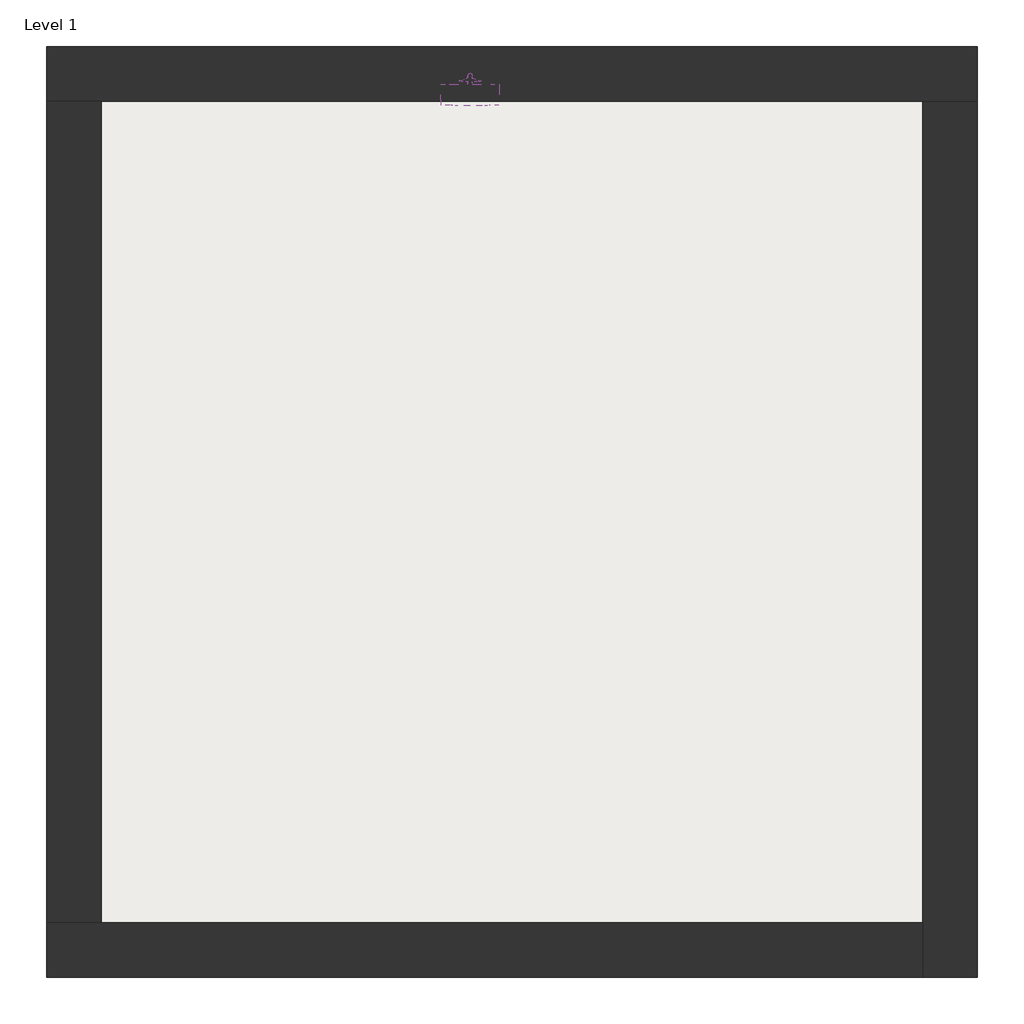
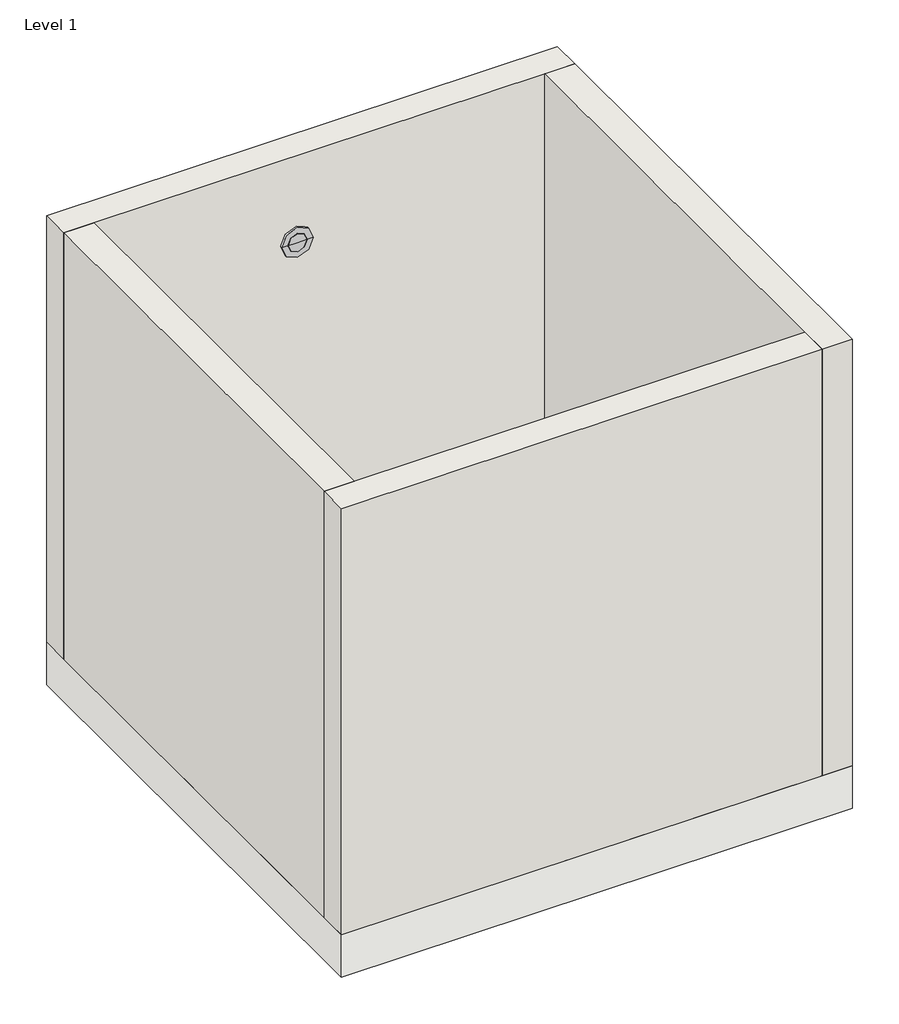
# One storey: 4 walls, 1 proxy, 1 slab.
"""IFC4 building model written with IfcOpenShell, lengths in millimetres."""

import ifcopenshell
import ifcopenshell.guid

model = None  # the IFC model being written
_history = None  # IfcOwnerHistory: only IFC2X3 demands one
_inside = {}  # id of a spatial element -> (the spatial element, [elements in it])
_under = {}  # id of a project, library or spatial element -> (it, [spatial elements below it])
_declared = {}  # id of a project -> (the project, [libraries it declares])
_typed = {}  # id of a type object -> (the type object, [elements of that type])
_made_of = {}  # id of a material, layer set ... -> (it, [elements and type objects made of it])


def new_model(schema):
    """Start an empty IFC model of exactly this schema.

    Asked for "IFC4X3", IfcOpenShell would pick the latest addendum, in which some entities
    have other attributes; the version numbers below select the first issue.
    IFC2X3 requires an IfcOwnerHistory on every rooted entity: one is made here for all.
    """
    global model, _history
    if schema == "IFC4X3":
        model = ifcopenshell.file(schema_version=(4, 3, 0, 0))
    else:
        model = ifcopenshell.file(schema=schema)
    _inside.clear()
    _under.clear()
    _declared.clear()
    _typed.clear()
    _made_of.clear()
    _history = None
    if model.schema == "IFC2X3":
        org = make("IfcOrganization", Name="unknown")
        user = make(
            "IfcPersonAndOrganization",
            ThePerson=make("IfcPerson", FamilyName="unknown"),
            TheOrganization=org,
        )
        app = make(
            "IfcApplication",
            ApplicationDeveloper=org,
            Version="unknown",
            ApplicationFullName="unknown",
            ApplicationIdentifier="unknown",
        )
        _history = make(
            "IfcOwnerHistory",
            OwningUser=user,
            OwningApplication=app,
            ChangeAction="ADDED",
            CreationDate=0,
        )
    return model


def make(cls, **values):
    """One entity of the class cls with the attributes given. An attribute that is None is left unset."""
    return model.create_entity(
        cls, **{name: value for name, value in values.items() if value is not None}
    )


def rooted(cls, **values):
    """An entity with a GlobalId (a new one), such as an element, a storey or a relation."""
    return make(cls, GlobalId=ifcopenshell.guid.new(), OwnerHistory=_history, **values)


def si_unit(unit_type, name, prefix=None):
    """IfcSIUnit, for example si_unit("LENGTHUNIT", "METRE", prefix="MILLI")."""
    return make("IfcSIUnit", UnitType=unit_type, Prefix=prefix, Name=name)


def assignment(units):
    """IfcUnitAssignment: the units of a project."""
    return None if units is None else make("IfcUnitAssignment", Units=units)


def point(xyz):
    """IfcCartesianPoint."""
    return None if xyz is None else make("IfcCartesianPoint", Coordinates=xyz)


def direction(xyz):
    """IfcDirection."""
    return None if xyz is None else make("IfcDirection", DirectionRatios=xyz)


def frame(location, z_axis=None, x_axis=None):
    """IfcAxis2Placement3D, a coordinate frame: its origin and axes. An axis left out is left unset."""
    return make(
        "IfcAxis2Placement3D",
        Location=point(location),
        Axis=direction(z_axis),
        RefDirection=direction(x_axis),
    )


def origin():
    """The frame at (0, 0, 0) with its axes left unset."""
    return frame((0.0, 0.0, 0.0))


def origin_with_axes():
    """The frame at (0, 0, 0) with the z axis (0, 0, 1) and the x axis (1, 0, 0) written out."""
    return frame((0.0, 0.0, 0.0), z_axis=(0.0, 0.0, 1.0), x_axis=(1.0, 0.0, 0.0))


def place(relative_to, where):
    """IfcLocalPlacement: puts the frame where relative to a parent placement (None: the world)."""
    return make(
        "IfcLocalPlacement", PlacementRelTo=relative_to, RelativePlacement=where
    )


def context(
    kind, dimensions, precision=None, world=None, true_north=None, identifier=None
):
    """IfcGeometricRepresentationContext, for example the 3D "Model" context."""
    return make(
        "IfcGeometricRepresentationContext",
        ContextIdentifier=identifier,
        ContextType=kind,
        CoordinateSpaceDimension=dimensions,
        Precision=precision,
        WorldCoordinateSystem=world,
        TrueNorth=true_north,
    )


def project(units=None, contexts=None):
    """IfcProject with its units and contexts."""
    return rooted(
        "IfcProject",
        Name="project",
        RepresentationContexts=contexts,
        UnitsInContext=assignment(units),
    )


def spatial(cls, under=None, at=None, **own):
    """A site, building, storey or space (cls), placed at a placement, below another one or the project."""
    s = rooted(cls, ObjectPlacement=at, **own)
    if under is not None:
        _under.setdefault(under.id(), (under, []))[1].append(s)
    return s


def polyline(points):
    """IfcPolyline through the points."""
    return make("IfcPolyline", Points=[point(p) for p in points])


def circle_curve(where, radius):
    """IfcCircle in the frame where."""
    return make("IfcCircle", Position=where, Radius=radius)


def ellipse_curve(where, semi_axis1, semi_axis2):
    """IfcEllipse in the frame where."""
    return make(
        "IfcEllipse", Position=where, SemiAxis1=semi_axis1, SemiAxis2=semi_axis2
    )


def trimmed(basis, trim1, trim2, sense, master):
    """IfcTrimmedCurve: the piece of a basis curve between two trims."""
    return make(
        "IfcTrimmedCurve",
        BasisCurve=basis,
        Trim1=trim1,
        Trim2=trim2,
        SenseAgreement=sense,
        MasterRepresentation=master,
    )


def outline(outer, holes=None, kind="AREA"):
    """IfcArbitraryClosedProfileDef: a profile drawn as a closed curve; with holes, ...WithVoids."""
    if holes is None:
        return make("IfcArbitraryClosedProfileDef", ProfileType=kind, OuterCurve=outer)
    return make(
        "IfcArbitraryProfileDefWithVoids",
        ProfileType=kind,
        OuterCurve=outer,
        InnerCurves=holes,
    )


def extrude(swept, where, along, depth):
    """IfcExtrudedAreaSolid: the profile swept, set in the frame where, extruded along a direction by depth."""
    return make(
        "IfcExtrudedAreaSolid",
        SweptArea=swept,
        Position=where,
        ExtrudedDirection=direction(along),
        Depth=depth,
    )


def faces_of(points, faces, orient=None, outer=None):
    """IfcFace entities. A face is a list of loops; a loop is a list of indices into points, from 0.

    orient and outer hold one flag for each loop. By default every Orientation is true, the
    first loop of a face is its IfcFaceOuterBound and the others are IfcFaceBound.
    """
    made = []
    for i, loops in enumerate(faces):
        bounds = []
        for j, loop in enumerate(loops):
            is_outer = j == 0 if outer is None else outer[i][j]
            bounds.append(
                make(
                    "IfcFaceOuterBound" if is_outer else "IfcFaceBound",
                    Bound=make("IfcPolyLoop", Polygon=[points[k] for k in loop]),
                    Orientation=True if orient is None else orient[i][j],
                )
            )
        made.append(make("IfcFace", Bounds=bounds))
    return made


def faceted_brep(points, faces, orient=None, outer=None, voids=None):
    """IfcFacetedBrep: a solid bounded by flat faces; with voids (closed shells), ...WithVoids."""
    shared = [point(p) for p in points]
    hull = make("IfcClosedShell", CfsFaces=faces_of(shared, faces, orient, outer))
    if voids is None:
        return make("IfcFacetedBrep", Outer=hull)
    return make(
        "IfcFacetedBrepWithVoids",
        Outer=hull,
        Voids=[
            make(cls, CfsFaces=faces_of(shared, fs, o, b)) for cls, fs, o, b in voids
        ],
    )


def shape(context_of_items, identifier, shape_type, items):
    """IfcShapeRepresentation: the items that make up one representation, for example the "Body"."""
    return make(
        "IfcShapeRepresentation",
        ContextOfItems=context_of_items,
        RepresentationIdentifier=identifier,
        RepresentationType=shape_type,
        Items=items,
    )


def source(mapping_origin, context_of_items, identifier, shape_type, items):
    """IfcRepresentationMap: a shape defined once, which mapped items show again and again."""
    return make(
        "IfcRepresentationMap",
        MappingOrigin=mapping_origin,
        MappedRepresentation=shape(context_of_items, identifier, shape_type, items),
    )


def transform(
    local_origin,
    x_axis=None,
    y_axis=None,
    z_axis=None,
    scale=None,
    scale2=None,
    scale3=None,
    uniform=True,
):
    """IfcCartesianTransformationOperator3D, or its non-uniform kind. x_axis, y_axis, z_axis: its Axis1, 2, 3."""
    if uniform:
        return make(
            "IfcCartesianTransformationOperator3D",
            Axis1=direction(x_axis),
            Axis2=direction(y_axis),
            LocalOrigin=point(local_origin),
            Scale=scale,
            Axis3=direction(z_axis),
        )
    return make(
        "IfcCartesianTransformationOperator3DnonUniform",
        Axis1=direction(x_axis),
        Axis2=direction(y_axis),
        LocalOrigin=point(local_origin),
        Scale=scale,
        Axis3=direction(z_axis),
        Scale2=scale2,
        Scale3=scale3,
    )


def mapped(mapping_source, mapping_target):
    """IfcMappedItem: shows the shape of a source again, moved by a transform."""
    return make(
        "IfcMappedItem", MappingSource=mapping_source, MappingTarget=mapping_target
    )


def made_of(thing, what):
    """Note that an element or type object is made of a material, layer set ...; save() writes the relation."""
    if what is not None:
        _made_of.setdefault(what.id(), (what, []))[1].append(thing)
    return thing


def element(
    cls,
    number,
    at=None,
    inside=None,
    cuts=None,
    type_object=None,
    material=None,
    context=None,
    identifier="Body",
    shape_type=None,
    held_by="IfcProductDefinitionShape",
    body=None,
    shapes=None,
    **own,
):
    """One element of the class cls, such as IfcWall. Its Tag is "e" and its number.

    at: its placement. inside: the storey or other place that contains it. cuts: it is an
    opening in that element (IfcRelVoidsElement). A single representation is given by context,
    identifier, shape_type and body (its items); several are given by shapes. held_by: the class
    of the entity that holds the representations. save() writes the other relations.
    """
    e = rooted(cls, Tag="e%d" % number, ObjectPlacement=at, **own)
    if body is not None:
        shapes = [shape(context, identifier, shape_type, body)]
    if shapes is not None:
        e.Representation = make(held_by, Representations=shapes)
    if inside is not None:
        _inside.setdefault(inside.id(), (inside, []))[1].append(e)
    if cuts is not None:
        rooted(
            "IfcRelVoidsElement", RelatingBuildingElement=cuts, RelatedOpeningElement=e
        )
    if type_object is not None:
        _typed.setdefault(type_object.id(), (type_object, []))[1].append(e)
    return made_of(e, material)


def aggregate(whole, parts):
    """IfcRelAggregates: a whole, such as a stair, and the parts it consists of."""
    return rooted("IfcRelAggregates", RelatingObject=whole, RelatedObjects=parts)


def save(model, path):
    """Write the relations noted so far, then the file.

    IfcRelAggregates (storeys below a building ...), IfcRelContainedInSpatialStructure (elements
    in a storey), IfcRelDefinesByType, IfcRelAssociatesMaterial and IfcRelDeclares: one each for
    every whole, place, type object, material and project.
    """
    for whole, parts in _under.values():
        aggregate(whole, parts)
    for where, things in _inside.values():
        rooted(
            "IfcRelContainedInSpatialStructure",
            RelatedElements=things,
            RelatingStructure=where,
        )
    for kind, things in _typed.values():
        rooted("IfcRelDefinesByType", RelatedObjects=things, RelatingType=kind)
    for what, things in _made_of.values():
        rooted("IfcRelAssociatesMaterial", RelatedObjects=things, RelatingMaterial=what)
    for by, libraries in _declared.values():
        rooted("IfcRelDeclares", RelatingContext=by, RelatedDefinitions=libraries)
    model.write(path)


def plane_surface(at):
    """IfcPlane: the flat surface through the origin of the frame at, square to its z axis."""
    return make("IfcPlane", Position=at)


def cylinder_surface(at, radius):
    """IfcCylindricalSurface: all points at the distance radius from the z axis of the frame at."""
    return make("IfcCylindricalSurface", Position=at, Radius=radius)


def revolved_surface(curve, axis_point, axis_direction):
    """IfcSurfaceOfRevolution: the curve turned about the line through axis_point along axis_direction."""
    return make(
        "IfcSurfaceOfRevolution",
        SweptCurve=make("IfcArbitraryOpenProfileDef", ProfileType="CURVE", Curve=curve),
        AxisPosition=make("IfcAxis1Placement", Location=point(axis_point), Axis=direction(axis_direction)),
    )


def spline_curve(degree, points, multiplicities, knots, weights=None):
    """IfcBSplineCurveWithKnots; with weights, IfcRationalBSplineCurveWithKnots."""
    own = dict(
        Degree=degree,
        ControlPointsList=[point(p) for p in points],
        CurveForm="UNSPECIFIED",
        ClosedCurve=False,
        SelfIntersect=False,
        KnotMultiplicities=multiplicities,
        Knots=knots,
        KnotSpec="UNSPECIFIED",
    )
    if weights is None:
        return make("IfcBSplineCurveWithKnots", **own)
    return make("IfcRationalBSplineCurveWithKnots", WeightsData=weights, **own)


def advanced_brep(points, edges, surfaces, faces):
    """IfcAdvancedBrep: a solid bounded by faces that lie on surfaces and meet in shared edges.

    An edge is (start, end): straight between two places in points (the first is 0);
    or (start, end, curve); or (start, end, curve, False) where it runs against its curve.
    A face is (place in surfaces, loops), or (place, loops, False) where it looks against
    its surface's normal. A loop lists edges by number (the first is 1), with a minus sign
    where the edge is run from its end to its start. The first loop is the outer one.
    """
    corners = [point(p) for p in points]
    vertices = [make("IfcVertexPoint", VertexGeometry=c) for c in corners]
    made = []
    for start, end, *more in edges:
        made.append(
            make(
                "IfcEdgeCurve",
                EdgeStart=vertices[start],
                EdgeEnd=vertices[end],
                EdgeGeometry=more[0] if more else make("IfcPolyline", Points=[corners[start], corners[end]]),
                SameSense=more[1] if len(more) > 1 else True,
            )
        )
    hull = []
    for where, loops, *sense in faces:
        bounds = []
        for j, loop in enumerate(loops):
            ring = [make("IfcOrientedEdge", EdgeElement=made[abs(k) - 1], Orientation=k > 0) for k in loop]
            bounds.append(
                make(
                    "IfcFaceOuterBound" if j == 0 else "IfcFaceBound",
                    Bound=make("IfcEdgeLoop", EdgeList=ring),
                    Orientation=True,
                )
            )
        hull.append(make("IfcAdvancedFace", Bounds=bounds, FaceSurface=surfaces[where], SameSense=sense[0] if sense else True))
    return make("IfcAdvancedBrep", Outer=make("IfcClosedShell", CfsFaces=hull))


def mechanical_equipment_c477e944(model_context):
    return source(origin(), model_context, "Body", "AdvancedBrep", [
        advanced_brep(
        [(121.9974459, -0.199999, 2400.0), (128.0025541, -0.199999, 2400.0), (128.0025541, -2.4999994, 2400.0), (121.9974459, -2.4999994, 2400.0), (119.1058972, -0.199999, 2400.0), (130.8941028, -0.199999, 2400.0), (119.1058972, 4.9999993, 2400.0), (130.8941028, 4.9999993, 2400.0), (116.7764643, 4.9999993, 2400.0), (133.2235357, 4.9999993, 2400.0), (116.7764643, 10.0000007, 2400.0), (133.2235357, 10.0000007, 2400.0), (117.7564219, 10.0000007, 2400.0), (132.2435781, 10.0000007, 2400.0), (117.7564219, 13.8000004, 2400.0), (132.2435781, 13.8000004, 2400.0), (116.0662237, 13.8000004, 2400.0), (133.9337763, 13.8000004, 2400.0), (114.7691944, 15.1302816, 2400.0), (135.2308056, 15.1302816, 2400.0), (114.7691944, 15.9854344, 2400.0), (135.2308056, 15.9854344, 2400.0), (111.2784266, 15.9854344, 2400.0), (138.7215734, 15.9854344, 2400.0), (90.472179, 26.7999995, 2400.0), (159.527821, 26.7999995, 2400.0), (87.519154, 26.7999995, 2400.0), (162.480846, 26.7999995, 2400.0), (86.2128962, 25.9940284, 2400.0), (163.7871038, 25.9940284, 2400.0), (86.2128962, 24.0999996, 2400.0), (163.7871038, 24.0999996, 2400.0), (85.0392013, 24.0999996, 2400.0), (164.9607987, 24.0999996, 2400.0), (85.0392013, 25.9940284, 2400.0), (164.9607987, 25.9940284, 2400.0), (87.0451729, 28.0, 2400.0), (162.9548271, 28.0, 2400.0), (119.1058972, 28.0, 2400.0), (130.8941028, 28.0, 2400.0), (119.1058972, 32.5000002, 2400.0), (130.8941028, 32.5000002, 2400.0), (116.7764643, 32.5000002, 2400.0), (133.2235357, 32.5000002, 2400.0), (116.7764643, 37.4999999, 2400.0), (133.2235357, 37.4999999, 2400.0), (18.250711, 37.4999999, 2400.0), (231.749289, 37.4999999, 2400.0), (19.5859291, 113.9945916, 2400.0), (230.4140709, 113.9945916, 2400.0), (59.5859291, 113.9945916, 2400.0), (190.4140709, 113.9945916, 2400.0), (61.724849, 116.1335115, 2400.0), (188.275151, 116.1335115, 2400.0), (125.0, 116.1335115, 2400.0), (125.0, -2.4999994, 2400.0)],
        [
            (0, 1, circle_curve(frame((125.0, -0.199999, 2400.0), z_axis=(0.0, -1.0, 0.0), x_axis=(1.0, 0.0, 0.0)), 3.0025541)),
            (1, 2),
            (2, 3, circle_curve(frame((125.0, -2.4999994, 2400.0), z_axis=(0.0, 1.0, 0.0), x_axis=(1.0, 0.0, 0.0)), 3.0025541)),
            (3, 0),
            (1, 0, circle_curve(frame((125.0, -0.199999, 2400.0), z_axis=(0.0, -1.0, 0.0), x_axis=(1.0, 0.0, 0.0)), 3.0025541)),
            (3, 2, circle_curve(frame((125.0, -2.4999994, 2400.0), z_axis=(0.0, 1.0, 0.0), x_axis=(1.0, 0.0, 0.0)), 3.0025541)),
            (4, 5, circle_curve(frame((125.0, -0.199999, 2400.0), z_axis=(0.0, -1.0, 0.0), x_axis=(1.0, 0.0, 0.0)), 5.8941028)),
            (5, 1),
            (0, 4),
            (5, 4, circle_curve(frame((125.0, -0.199999, 2400.0), z_axis=(0.0, -1.0, 0.0), x_axis=(1.0, 0.0, 0.0)), 5.8941028)),
            (6, 7, circle_curve(frame((125.0, 4.9999993, 2400.0), z_axis=(0.0, -1.0, 0.0), x_axis=(1.0, 0.0, 0.0)), 5.8941028)),
            (7, 5),
            (4, 6),
            (7, 6, circle_curve(frame((125.0, 4.9999993, 2400.0), z_axis=(0.0, -1.0, 0.0), x_axis=(1.0, 0.0, 0.0)), 5.8941028)),
            (8, 9, circle_curve(frame((125.0, 4.9999993, 2400.0), z_axis=(0.0, -1.0, 0.0), x_axis=(1.0, 0.0, 0.0)), 8.2235357)),
            (9, 7),
            (6, 8),
            (9, 8, circle_curve(frame((125.0, 4.9999993, 2400.0), z_axis=(0.0, -1.0, 0.0), x_axis=(1.0, 0.0, 0.0)), 8.2235357)),
            (10, 11, circle_curve(frame((125.0, 10.0000007, 2400.0), z_axis=(0.0, -1.0, 0.0), x_axis=(1.0, 0.0, 0.0)), 8.2235357)),
            (11, 9),
            (8, 10),
            (11, 10, circle_curve(frame((125.0, 10.0000007, 2400.0), z_axis=(0.0, -1.0, 0.0), x_axis=(1.0, 0.0, 0.0)), 8.2235357)),
            (12, 13, circle_curve(frame((125.0, 10.0000007, 2400.0), z_axis=(0.0, -1.0, 0.0), x_axis=(1.0, 0.0, 0.0)), 7.2435781)),
            (13, 11),
            (10, 12),
            (13, 12, circle_curve(frame((125.0, 10.0000007, 2400.0), z_axis=(0.0, -1.0, 0.0), x_axis=(1.0, 0.0, 0.0)), 7.2435781)),
            (14, 15, circle_curve(frame((125.0, 13.8000004, 2400.0), z_axis=(0.0, -1.0, 0.0), x_axis=(1.0, 0.0, 0.0)), 7.2435781)),
            (15, 13),
            (12, 14),
            (15, 14, circle_curve(frame((125.0, 13.8000004, 2400.0), z_axis=(0.0, -1.0, 0.0), x_axis=(1.0, 0.0, 0.0)), 7.2435781)),
            (16, 17, circle_curve(frame((125.0, 13.8000004, 2400.0), z_axis=(0.0, -1.0, 0.0), x_axis=(1.0, 0.0, 0.0)), 8.9337763)),
            (17, 15),
            (14, 16),
            (17, 16, circle_curve(frame((125.0, 13.8000004, 2400.0), z_axis=(0.0, -1.0, 0.0), x_axis=(1.0, 0.0, 0.0)), 8.9337763)),
            (18, 19, circle_curve(frame((125.0, 15.1302816, 2400.0), z_axis=(0.0, -1.0, 0.0), x_axis=(1.0, 0.0, 0.0)), 10.2308056)),
            (19, 17, spline_curve(3, [(135.2308056, 15.1302816, 2400.0), (135.18031757, 14.408269131, 2400.0), (134.747974442, 13.964842091, 2400.0), (133.9337763, 13.8000004, 2400.0)], [4, 4], [0.0, 0.003825031864308585])),
            (16, 18, spline_curve(3, [(116.0662237, 13.8000004, 2400.0), (115.252025558, 13.964842091, 2400.0), (114.81968243, 14.408269131, 2400.0), (114.7691944, 15.1302816, 2400.0)], [4, 4], [0.0, 0.003825031864308585])),
            (19, 18, circle_curve(frame((125.0, 15.1302816, 2400.0), z_axis=(0.0, -1.0, 0.0), x_axis=(1.0, 0.0, 0.0)), 10.2308056)),
            (20, 21, circle_curve(frame((125.0, 15.9854344, 2400.0), z_axis=(0.0, -1.0, 0.0), x_axis=(1.0, 0.0, 0.0)), 10.2308056)),
            (21, 19),
            (18, 20),
            (21, 20, circle_curve(frame((125.0, 15.9854344, 2400.0), z_axis=(0.0, -1.0, 0.0), x_axis=(1.0, 0.0, 0.0)), 10.2308056)),
            (22, 23, circle_curve(frame((125.0, 15.9854344, 2400.0), z_axis=(0.0, -1.0, 0.0), x_axis=(1.0, 0.0, 0.0)), 13.7215734)),
            (23, 21),
            (20, 22),
            (23, 22, circle_curve(frame((125.0, 15.9854344, 2400.0), z_axis=(0.0, -1.0, 0.0), x_axis=(1.0, 0.0, 0.0)), 13.7215734)),
            (24, 25, circle_curve(frame((125.0, 26.7999995, 2400.0), z_axis=(0.0, -1.0, 0.0), x_axis=(1.0, 0.0, 0.0)), 34.527821)),
            (25, 23, spline_curve(3, [(159.527821, 26.7999995, 2400.0), (152.920328589, 20.192507089, 2400.0), (145.984912731, 16.587652064, 2400.0), (138.7215734, 15.9854344, 2400.0)], [4, 4], [0.0, 0.04037262450680565])),
            (22, 24, spline_curve(3, [(111.2784266, 15.9854344, 2400.0), (104.015087269, 16.587652064, 2400.0), (97.079671411, 20.192507089, 2400.0), (90.472179, 26.7999995, 2400.0)], [4, 4], [0.0, 0.04037262450680565])),
            (25, 24, circle_curve(frame((125.0, 26.7999995, 2400.0), z_axis=(0.0, -1.0, 0.0), x_axis=(1.0, 0.0, 0.0)), 34.527821)),
            (26, 27, circle_curve(frame((125.0, 26.7999995, 2400.0), z_axis=(0.0, -1.0, 0.0), x_axis=(1.0, 0.0, 0.0)), 37.480846)),
            (27, 25),
            (24, 26),
            (27, 26, circle_curve(frame((125.0, 26.7999995, 2400.0), z_axis=(0.0, -1.0, 0.0), x_axis=(1.0, 0.0, 0.0)), 37.480846)),
            (28, 29, circle_curve(frame((125.0, 25.9940284, 2400.0), z_axis=(0.0, -1.0, 0.0), x_axis=(1.0, 0.0, 0.0)), 38.7871038)),
            (29, 27, circle_curve(frame((162.7127782, 25.7143697, 2400.0), z_axis=(0.0, 0.0, 1.0), x_axis=(-1.0, 0.0, 0.0)), 1.1101281)),
            (26, 28, circle_curve(frame((87.2872218, 25.7143697, 2400.0), z_axis=(0.0, 0.0, 1.0), x_axis=(1.0, 0.0, 0.0)), 1.1101281)),
            (29, 28, circle_curve(frame((125.0, 25.9940284, 2400.0), z_axis=(0.0, -1.0, 0.0), x_axis=(1.0, 0.0, 0.0)), 38.7871038)),
            (30, 31, circle_curve(frame((125.0, 24.0999996, 2400.0), z_axis=(0.0, -1.0, 0.0), x_axis=(1.0, 0.0, 0.0)), 38.7871038)),
            (31, 29),
            (28, 30),
            (31, 30, circle_curve(frame((125.0, 24.0999996, 2400.0), z_axis=(0.0, -1.0, 0.0), x_axis=(1.0, 0.0, 0.0)), 38.7871038)),
            (32, 33, circle_curve(frame((125.0, 24.0999996, 2400.0), z_axis=(0.0, -1.0, 0.0), x_axis=(1.0, 0.0, 0.0)), 39.9607987)),
            (33, 31),
            (30, 32),
            (33, 32, circle_curve(frame((125.0, 24.0999996, 2400.0), z_axis=(0.0, -1.0, 0.0), x_axis=(1.0, 0.0, 0.0)), 39.9607987)),
            (34, 35, circle_curve(frame((125.0, 25.9940284, 2400.0), z_axis=(0.0, -1.0, 0.0), x_axis=(1.0, 0.0, 0.0)), 39.9607987)),
            (35, 33),
            (32, 34),
            (35, 34, circle_curve(frame((125.0, 25.9940284, 2400.0), z_axis=(0.0, -1.0, 0.0), x_axis=(1.0, 0.0, 0.0)), 39.9607987)),
            (36, 37, circle_curve(frame((125.0, 28.0, 2400.0), z_axis=(0.0, -1.0, 0.0), x_axis=(1.0, 0.0, 0.0)), 37.9548271)),
            (37, 35, circle_curve(frame((162.9548271, 25.9940284, 2400.0), z_axis=(0.0, 0.0, -1.0), x_axis=(-1.0, 0.0, 0.0)), 2.0059716)),
            (34, 36, circle_curve(frame((87.0451729, 25.9940284, 2400.0), z_axis=(0.0, 0.0, -1.0), x_axis=(1.0, 0.0, 0.0)), 2.0059716)),
            (37, 36, circle_curve(frame((125.0, 28.0, 2400.0), z_axis=(0.0, -1.0, 0.0), x_axis=(1.0, 0.0, 0.0)), 37.9548271)),
            (38, 39, circle_curve(frame((125.0, 28.0, 2400.0), z_axis=(0.0, -1.0, 0.0), x_axis=(1.0, 0.0, 0.0)), 5.8941028)),
            (39, 37),
            (36, 38),
            (39, 38, circle_curve(frame((125.0, 28.0, 2400.0), z_axis=(0.0, -1.0, 0.0), x_axis=(1.0, 0.0, 0.0)), 5.8941028)),
            (40, 41, circle_curve(frame((125.0, 32.5000002, 2400.0), z_axis=(0.0, -1.0, 0.0), x_axis=(1.0, 0.0, 0.0)), 5.8941028)),
            (41, 39),
            (38, 40),
            (41, 40, circle_curve(frame((125.0, 32.5000002, 2400.0), z_axis=(0.0, -1.0, 0.0), x_axis=(1.0, 0.0, 0.0)), 5.8941028)),
            (42, 43, circle_curve(frame((125.0, 32.5000002, 2400.0), z_axis=(0.0, -1.0, 0.0), x_axis=(1.0, 0.0, 0.0)), 8.2235357)),
            (43, 41),
            (40, 42),
            (43, 42, circle_curve(frame((125.0, 32.5000002, 2400.0), z_axis=(0.0, -1.0, 0.0), x_axis=(1.0, 0.0, 0.0)), 8.2235357)),
            (44, 45, circle_curve(frame((125.0, 37.4999999, 2400.0), z_axis=(0.0, -1.0, 0.0), x_axis=(1.0, 0.0, 0.0)), 8.2235357)),
            (45, 43),
            (42, 44),
            (45, 44, circle_curve(frame((125.0, 37.4999999, 2400.0), z_axis=(0.0, -1.0, 0.0), x_axis=(1.0, 0.0, 0.0)), 8.2235357)),
            (46, 47, circle_curve(frame((125.0, 37.4999999, 2400.0), z_axis=(0.0, -1.0, 0.0), x_axis=(1.0, 0.0, 0.0)), 106.749289)),
            (47, 45),
            (44, 46),
            (47, 46, circle_curve(frame((125.0, 37.4999999, 2400.0), z_axis=(0.0, -1.0, 0.0), x_axis=(1.0, 0.0, 0.0)), 106.749289)),
            (48, 49, circle_curve(frame((125.0, 113.9945916, 2400.0), z_axis=(0.0, -1.0, 0.0), x_axis=(1.0, 0.0, 0.0)), 105.4140709)),
            (49, 47),
            (46, 48),
            (49, 48, circle_curve(frame((125.0, 113.9945916, 2400.0), z_axis=(0.0, -1.0, 0.0), x_axis=(1.0, 0.0, 0.0)), 105.4140709)),
            (50, 51, circle_curve(frame((125.0, 113.9945916, 2400.0), z_axis=(0.0, -1.0, 0.0), x_axis=(1.0, 0.0, 0.0)), 65.4140709)),
            (51, 49),
            (48, 50),
            (51, 50, circle_curve(frame((125.0, 113.9945916, 2400.0), z_axis=(0.0, -1.0, 0.0), x_axis=(1.0, 0.0, 0.0)), 65.4140709)),
            (52, 53, circle_curve(frame((125.0, 116.1335115, 2400.0), z_axis=(0.0, -1.0, 0.0), x_axis=(1.0, 0.0, 0.0)), 63.275151)),
            (53, 51),
            (50, 52),
            (53, 52, circle_curve(frame((125.0, 116.1335115, 2400.0), z_axis=(0.0, -1.0, 0.0), x_axis=(1.0, 0.0, 0.0)), 63.275151)),
            (54, 53),
            (52, 54),
            (2, 55),
            (55, 3),
        ],
        [
            cylinder_surface(frame((125.0, -65.0, 2400.0), z_axis=(0.0, 1.0, 0.0), x_axis=(1.0, 0.0, 0.0)), 3.0025541),
            plane_surface(frame((125.0, -0.199999, 2400.0), z_axis=(0.0, -1.0, 0.0), x_axis=(1.0, 0.0, 0.0))),
            cylinder_surface(frame((125.0, -65.0, 2400.0), z_axis=(0.0, 1.0, 0.0), x_axis=(1.0, 0.0, 0.0)), 5.8941028),
            plane_surface(frame((125.0, 4.9999993, 2400.0), z_axis=(0.0, -1.0, 0.0), x_axis=(1.0, 0.0, 0.0))),
            cylinder_surface(frame((125.0, -65.0, 2400.0), z_axis=(0.0, 1.0, 0.0), x_axis=(1.0, 0.0, 0.0)), 8.2235357),
            plane_surface(frame((125.0, 10.0000007, 2400.0), z_axis=(0.0, 1.0, 0.0), x_axis=(1.0, 0.0, 0.0))),
            cylinder_surface(frame((125.0, -65.0, 2400.0), z_axis=(0.0, 1.0, 0.0), x_axis=(1.0, 0.0, 0.0)), 7.2435781),
            plane_surface(frame((125.0, 13.8000004, 2400.0), z_axis=(0.0, -1.0, 0.0), x_axis=(1.0, 0.0, 0.0))),
            revolved_surface(spline_curve(3, [(133.9337763, 13.8000004, 2400.0), (134.747974442, 13.964842091, 2400.0), (135.18031757, 14.408269131, 2400.0), (135.2308056, 15.1302816, 2400.0)], [4, 4], [0.0, 0.003825031864308585]), (125.0, -65.0, 2400.0), (0.0, 1.0, 0.0)),
            cylinder_surface(frame((125.0, -65.0, 2400.0), z_axis=(0.0, 1.0, 0.0), x_axis=(1.0, 0.0, 0.0)), 10.2308056),
            plane_surface(frame((125.0, 15.9854344, 2400.0), z_axis=(0.0, -1.0, 0.0), x_axis=(1.0, 0.0, 0.0))),
            revolved_surface(spline_curve(3, [(138.7215734, 15.9854344, 2400.0), (145.984912731, 16.587652064, 2400.0), (152.920328589, 20.192507089, 2400.0), (159.527821, 26.7999995, 2400.0)], [4, 4], [0.0, 0.04037262450680565]), (125.0, -65.0, 2400.0), (0.0, 1.0, 0.0)),
            plane_surface(frame((125.0, 26.7999995, 2400.0), z_axis=(0.0, -1.0, 0.0), x_axis=(1.0, 0.0, 0.0))),
            revolved_surface(trimmed(ellipse_curve(frame((162.7127782, 25.7143697, 2400.0), z_axis=(0.0, 0.0, -1.0), x_axis=(-1.0, 0.0, 0.0)), 1.1101281, 1.1101281), [point((162.480846, 26.7999995, 2400.0))], [point((163.7871038, 25.9940284, 2400.0))], True, "CARTESIAN"), (125.0, -65.0, 2400.0), (0.0, 1.0, 0.0)),
            revolved_surface(polyline([(163.7871038, 25.994028400000005, 2400.0), (163.7871038, 24.099999600000004, 2400.0)]), (125.0, -65.0, 2400.0), (0.0, 1.0, 0.0)),
            plane_surface(frame((125.0, 24.0999996, 2400.0), z_axis=(0.0, -1.0, 0.0), x_axis=(1.0, 0.0, 0.0))),
            cylinder_surface(frame((125.0, -65.0, 2400.0), z_axis=(0.0, 1.0, 0.0), x_axis=(1.0, 0.0, 0.0)), 39.9607987),
            revolved_surface(trimmed(ellipse_curve(frame((162.9548271, 25.9940284, 2400.0), z_axis=(0.0, 0.0, 1.0), x_axis=(-1.0, 0.0, 0.0)), 2.0059716, 2.0059716), [point((164.9607987, 25.9940284, 2400.0))], [point((162.9548271, 28.0, 2400.0))], True, "CARTESIAN"), (125.0, -65.0, 2400.0), (0.0, 1.0, 0.0)),
            plane_surface(frame((125.0, 28.0, 2400.0), z_axis=(0.0, 1.0, 0.0), x_axis=(1.0, 0.0, 0.0))),
            plane_surface(frame((125.0, 32.5000002, 2400.0), z_axis=(0.0, -1.0, 0.0), x_axis=(1.0, 0.0, 0.0))),
            plane_surface(frame((125.0, 37.4999999, 2400.0), z_axis=(0.0, -1.0, 0.0), x_axis=(1.0, 0.0, 0.0))),
            revolved_surface(polyline([(231.749289, 37.4999999, 2400.0), (230.4140709, 113.9945916, 2400.0)]), (125.0, -65.0, 2400.0), (0.0, 1.0, 0.0)),
            plane_surface(frame((125.0, 113.9945916, 2400.0), z_axis=(0.0, 1.0, 0.0), x_axis=(1.0, 0.0, 0.0))),
            revolved_surface(polyline([(190.4140709, 113.9945916, 2400.0), (188.275151, 116.1335115, 2400.0)]), (125.0, -65.0, 2400.0), (0.0, 1.0, 0.0)),
            plane_surface(frame((125.0, 116.1335115, 2400.0), z_axis=(0.0, 1.0, 0.0), x_axis=(1.0, 0.0, 0.0))),
            plane_surface(frame((125.0, -2.4999994, 2400.0), z_axis=(0.0, -1.0, 0.0), x_axis=(1.0, 0.0, 0.0))),
        ],
        [
            (0, [[1, 2, 3, 4]]),
            (0, [[5, -4, 6, -2]]),
            (1, [[7, 8, -1, 9]]),
            (1, [[10, -9, -5, -8]]),
            (2, [[11, 12, -7, 13]]),
            (2, [[14, -13, -10, -12]]),
            (3, [[15, 16, -11, 17]]),
            (3, [[18, -17, -14, -16]]),
            (4, [[19, 20, -15, 21]]),
            (4, [[22, -21, -18, -20]]),
            (5, [[23, 24, -19, 25]]),
            (5, [[26, -25, -22, -24]]),
            (6, [[27, 28, -23, 29]]),
            (6, [[30, -29, -26, -28]]),
            (7, [[31, 32, -27, 33]]),
            (7, [[34, -33, -30, -32]]),
            (8, [[35, 36, -31, 37]]),
            (8, [[38, -37, -34, -36]]),
            (9, [[39, 40, -35, 41]]),
            (9, [[42, -41, -38, -40]]),
            (10, [[43, 44, -39, 45]]),
            (10, [[46, -45, -42, -44]]),
            (11, [[47, 48, -43, 49]]),
            (11, [[50, -49, -46, -48]]),
            (12, [[51, 52, -47, 53]]),
            (12, [[54, -53, -50, -52]]),
            (13, [[55, 56, -51, 57]]),
            (13, [[58, -57, -54, -56]]),
            (14, [[59, 60, -55, 61]]),
            (14, [[62, -61, -58, -60]]),
            (15, [[63, 64, -59, 65]]),
            (15, [[66, -65, -62, -64]]),
            (16, [[67, 68, -63, 69]]),
            (16, [[70, -69, -66, -68]]),
            (17, [[71, 72, -67, 73]]),
            (17, [[74, -73, -70, -72]]),
            (18, [[75, 76, -71, 77]]),
            (18, [[78, -77, -74, -76]]),
            (2, [[79, 80, -75, 81]]),
            (2, [[82, -81, -78, -80]]),
            (19, [[83, 84, -79, 85]]),
            (19, [[86, -85, -82, -84]]),
            (4, [[87, 88, -83, 89]]),
            (4, [[90, -89, -86, -88]]),
            (20, [[91, 92, -87, 93]]),
            (20, [[94, -93, -90, -92]]),
            (21, [[95, 96, -91, 97]]),
            (21, [[98, -97, -94, -96]]),
            (22, [[99, 100, -95, 101]]),
            (22, [[102, -101, -98, -100]]),
            (23, [[103, 104, -99, 105]]),
            (23, [[106, -105, -102, -104]]),
            (24, [[107, -103, 108]]),
            (24, [[-108, -106, -107]]),
            (25, [[-3, 109, 110]]),
            (25, [[-6, -110, -109]]),
        ],
    ),
    ])


model = new_model("IFC4")

# Units and contexts
model_context = context("Model", 3, world=origin())
ifc_project = project(units=[si_unit("LENGTHUNIT", "METRE", prefix="MILLI")], contexts=[model_context])

# Site, building, storey
site = spatial("IfcSite", under=ifc_project)
building = spatial("IfcBuilding", under=site)
storey = spatial("IfcBuildingStorey", under=building, Name="Level 1", Elevation=0.0)

# Proxy
placement = place(None, origin())
mechanical_equipment_shape = mechanical_equipment_c477e944(model_context)
element("IfcBuildingElementProxy", 1, Name="BVNO 50 4L : BVNO 50 4L", ObjectType="BVNO 50 4L : BVNO 50 4L", at=placement, inside=storey, context=model_context, shape_type="MappedRepresentation", body=[
    mapped(mechanical_equipment_shape, transform((-9449.5629456, 11113.1412882, 0.0), x_axis=(-1.0, 0.0, 0.0), y_axis=(0.0, -1.0, 0.0), z_axis=(0.0, 0.0, 1.0))),
])

# Slab
element("IfcSlab", 2, ObjectType="Generic 300mm", at=placement, inside=storey, context=model_context, shape_type="SweptSolid", body=[
    extrude(outline(polyline([(-7721.3122346, 11213.1412882), (-7721.3122346, 7813.1412882), (-11121.3122346, 7813.1412882), (-11121.3122346, 11213.1412882), (-7721.3122346, 11213.1412882)])), frame((0.0, 0.0, -300.0), z_axis=(0.0, 0.0, 1.0), x_axis=(1.0, 0.0, 0.0)), (0.0, 0.0, 1.0), 300.0),
])

# Walls
element("IfcWall", 3, ObjectType="Generic - 200mm", at=placement, inside=storey, context=model_context, shape_type="Brep", body=[
    faceted_brep([(-11121.3122346, 11013.1412882, 0.0), (-10921.3122346, 11013.1412882, 0.0), (-7921.3122346, 11013.1412882, 0.0), (-7721.3122346, 11013.1412882, 0.0), (-7721.3122346, 11013.1412882, 3000.0), (-7921.3122346, 11013.1412882, 3000.0), (-10921.3122346, 11013.1412882, 3000.0), (-11121.3122346, 11013.1412882, 3000.0), (-11121.3122346, 11213.1412882, 0.0), (-11121.3122346, 11213.1412882, 3000.0), (-7721.3122346, 11213.1412882, 3000.0), (-7721.3122346, 11213.1412882, 0.0)], [[[0, 1, 2, 3, 4, 5, 6, 7]], [[8, 9, 10, 11]], [[3, 2, 1, 0, 8, 11]], [[7, 6, 5, 4, 10, 9]], [[4, 3, 11, 10]], [[0, 7, 9, 8]]]),
])
element("IfcWall", 4, ObjectType="Generic - 200mm", at=placement, inside=storey, context=model_context, shape_type="Brep", body=[
    faceted_brep([(-7921.3122346, 11013.1412882, 0.0), (-7921.3122346, 8013.1412882, 0.0), (-7921.3122346, 7813.1412882, 0.0), (-7921.3122346, 7813.1412882, 3000.0), (-7921.3122346, 8013.1412882, 3000.0), (-7921.3122346, 11013.1412882, 3000.0), (-7721.3122346, 11013.1412882, 0.0), (-7721.3122346, 11013.1412882, 3000.0), (-7721.3122346, 7813.1412882, 3000.0), (-7721.3122346, 7813.1412882, 0.0)], [[[0, 1, 2, 3, 4, 5]], [[6, 7, 8, 9]], [[2, 1, 0, 6, 9]], [[5, 4, 3, 8, 7]], [[0, 5, 7, 6]], [[3, 2, 9, 8]]]),
])
element("IfcWall", 5, ObjectType="Generic - 200mm", at=placement, inside=storey, context=model_context, shape_type="Brep", body=[
    faceted_brep([(-7921.3122346, 8013.1412882, 0.0), (-10921.3122346, 8013.1412882, 0.0), (-11121.3122346, 8013.1412882, 0.0), (-11121.3122346, 8013.1412882, 3000.0), (-10921.3122346, 8013.1412882, 3000.0), (-7921.3122346, 8013.1412882, 3000.0), (-7921.3122346, 7813.1412882, 0.0), (-7921.3122346, 7813.1412882, 3000.0), (-11121.3122346, 7813.1412882, 3000.0), (-11121.3122346, 7813.1412882, 0.0)], [[[0, 1, 2, 3, 4, 5]], [[6, 7, 8, 9]], [[2, 1, 0, 6, 9]], [[5, 4, 3, 8, 7]], [[0, 5, 7, 6]], [[3, 2, 9, 8]]]),
])
element("IfcWall", 6, ObjectType="Generic - 200mm", at=placement, inside=storey, context=model_context, shape_type="SweptSolid", body=[
    extrude(outline(polyline([(-10921.3122346, 11013.1412882), (-10921.3122346, 8013.1412882), (-11121.3122346, 8013.1412882), (-11121.3122346, 11013.1412882), (-10921.3122346, 11013.1412882)])), origin_with_axes(), (0.0, 0.0, 1.0), 3000.0),
])

save(model, "model.ifc")

# Revit data of these elements
# Project information
#   Project Issue Date = "Issue Date"
#   Project Status = "Project Status"
#   Client Name = "Owner"
#   Project Address = "Enter address here"
#   Project Name = "Project Name"
#   Project Number = "Project Number"
# Type "BVNO 50 4L : BVNO 50 4L"
#   Model = "BVNO 50 4L"
#   FLANGE HEIGHT [instance default] = 2400 mm
#   Default Elevation = 0
# Type "Generic 300mm"
#   Function = 0
#   Layers, outside or top first: 300 mm no material (function 1)
# Type "Generic - 200mm"
#   Layers, outside or top first: 200 mm no material (function 1)
# Element 1 (IfcBuildingElementProxy, "BVNO 50 4L : BVNO 50 4L")
#   Mark = "16"
#   FLANGE HEIGHT = 2400 mm
#   Phase Created = New Construction
# Element 2 (IfcSlab, "Generic 300mm")
#   Height Offset From Level = 0 mm
#   Phase Created = New Construction
#   Materials on its faces: "Default Floor"
# Elements 3, 4, 5, 6 (IfcWall, "Generic - 200mm")
#   Top Offset = 0 mm
#   Base Offset = 0 mm
#   Unconnected Height = 3000 mm
#   wall height = 3000 mm
#   Phase Created = New Construction
#   Base Constraint = Level 1
#   Materials on its faces: "Default Wall"
# Materials
#   "Default Floor": class "Miscellaneous", colour RGB 127 127 127, transparency 0, Cost = 0
#   "Default Wall": class "Miscellaneous", colour RGB 128 128 128, transparency 0, Cost = 0
